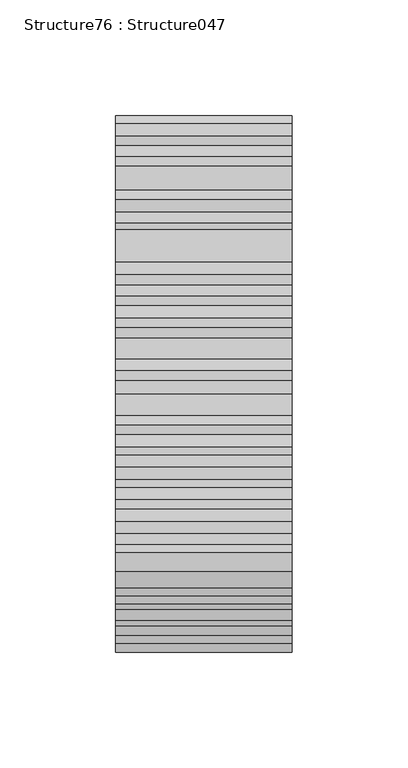
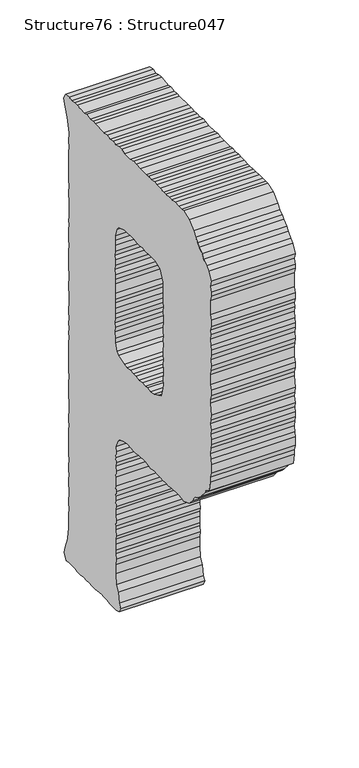
"""IFC4 building model written with IfcOpenShell, lengths in millimetres: proxy geometry, Structure76 : Structure047."""

from ifc_helpers import new_model, si_unit, frame, origin, place, context, project, spatial, polyline, outline, extrude, source, transform, mapped, element, save


def structure76_structure047_63e31db1(model_context):
    return source(origin(), model_context, "Body", "SweptSolid", [
        extrude(outline(polyline([(281300.9122556, 3996.390138), (281309.7038837, 3996.390138), (281314.3877242, 3997.5486624), (281318.4971163, 3997.5486624), (281323.7634282, 3996.390138), (281327.8647973, 3996.9645864), (281332.5566609, 3996.390138), (281337.2405014, 3996.9645864), (281342.5068134, 3996.390138), (281356.5663579, 3996.390138), (281359.5092026, 3996.9645864), (281364.1834155, 3996.390138), (281369.4673781, 3997.5486624), (281373.5687472, 3996.390138), (281384.1109987, 3997.5486624), (281388.2107632, 3997.5486624), (281392.9026268, 3996.390138), (281397.0039958, 3997.5486624), (281402.2703078, 3996.9645864), (281405.7876009, 3991.6806238), (281404.038582, 3986.4046842), (281402.2703078, 3982.8793681), (281401.0957373, 3978.2035506), (281399.3451138, 3973.5197101), (281397.0039958, 3962.9774586), (281398.1705433, 3954.7506513), (281397.0039958, 3948.917914), (281398.1705433, 3944.8165449), (281398.1705433, 3935.4328178), (281397.5864673, 3931.3346579), (281397.5864673, 3921.3748778), (281398.1705433, 3917.2735087), (281397.0039958, 3912.0071968), (281397.5864673, 3906.7328618), (281397.5864673, 3903.2059411), (281397.0039958, 3898.5301236), (281397.0039958, 3883.2863809), (281397.5864673, 3879.1769888), (281397.0039958, 3875.0772243), (281398.1705433, 3870.4030114), (281397.5864673, 3864.5446004), (281398.1705433, 3860.4432313), (281397.0039958, 3855.1769193), (281397.5864673, 3851.0595042), (281397.5864673, 3832.8921721), (281397.0039958, 3828.2163546), (281397.0039958, 3823.5341187), (281397.5864673, 3818.8310229), (281398.1705433, 3812.9726119), (281397.0039958, 3808.8888934), (281397.0039958, 3800.0876378), (281397.5864673, 3794.2292268), (281398.1705433, 3790.7039107), (281397.0039958, 3786.0280932), (281398.1705433, 3780.1616592), (281397.0039958, 3776.0618947), (281398.1705433, 3771.3860772), (281397.0039958, 3766.684586), (281397.5864673, 3762.0023501), (281397.5864673, 3756.7440611), (281398.1705433, 3752.6170184), (281398.1705433, 3743.2332913), (281397.5864673, 3739.1592005), (281398.1705433, 3733.8736333), (281397.0039958, 3729.7738688), (281397.5864673, 3723.9154578), (281397.5864673, 3720.4158154), (281398.1705433, 3715.1302482), (281397.5864673, 3709.8559132), (281397.0039958, 3705.7545441), (281397.0039958, 3696.9709391), (281397.5864673, 3691.0868544), (281397.5864673, 3686.4030139), (281397.0039958, 3682.8857208), (281397.5864673, 3678.2018803), (281398.1705433, 3672.9435914), (281397.5864673, 3668.8261762), (281397.5864673, 3662.9854159), (281398.1705433, 3658.3015753), (281398.1705433, 3654.1841602), (281397.0039958, 3650.1004418), (281398.1705433, 3644.2420307), (281397.5864673, 3639.5405396), (281397.0039958, 3635.4407751), (281397.5864673, 3630.7392839), (281397.5864673, 3626.6571701), (281397.0039958, 3620.7971545), (281397.0039958, 3616.0972679), (281398.1705433, 3612.0135494), (281398.1705433, 3607.8961343), (281397.0039958, 3602.6298224), (281398.1705433, 3597.9540049), (281398.1705433, 3593.8285667), (281397.5864673, 3588.5702778), (281397.5864673, 3584.4689087), (281399.3451138, 3573.9266571), (281399.9372129, 3570.4109687), (281402.2703078, 3564.54293), (281404.038582, 3559.8671125), (281405.1955018, 3556.3417965), (281401.6878364, 3550.4833855), (281397.5864673, 3551.0658569), (281387.6282918, 3551.0658569), (281384.1109987, 3550.4833855), (281379.4191352, 3550.4833855), (281374.1512186, 3551.0658569), (281369.4673781, 3550.4833855), (281365.3595906, 3551.0658569), (281360.6757501, 3550.4833855), (281356.5663579, 3550.4833855), (281346.0241064, 3551.6675836), (281342.5068134, 3551.6675836), (281338.4070489, 3551.0658569), (281333.1391323, 3550.4833855), (281323.1713292, 3550.4833855), (281318.4971163, 3551.6675836), (281316.1463707, 3556.3417965), (281318.4971163, 3559.8671125), (281320.2477398, 3569.2524442), (281323.1713292, 3575.0851816), (281324.3475043, 3584.4689087), (281324.3475043, 3593.2541183), (281323.1713292, 3599.1125293), (281324.3475043, 3603.7963698), (281323.7634282, 3607.3393366), (281324.3475043, 3613.1720739), (281324.3475043, 3617.8559144), (281323.1713292, 3621.3732075), (281324.3475043, 3626.6571701), (281323.7634282, 3630.7392839), (281323.1713292, 3636.0408972), (281324.3475043, 3640.7167147), (281324.3475043, 3645.9830266), (281323.1713292, 3649.5003197), (281323.7634282, 3654.7842823), (281323.7634282, 3659.4584952), (281323.1713292, 3664.1423357), (281323.7634282, 3668.8261762), (281323.7634282, 3677.6274319), (281323.1713292, 3683.4858429), (281324.3475043, 3687.587212), (281323.1713292, 3691.6869765), (281323.7634282, 3696.3884676), (281323.1713292, 3702.229228), (281324.3475043, 3706.3289925), (281320.8302112, 3713.9556777), (281318.4971163, 3716.8985223), (281310.8720357, 3719.2316172), (281305.0120201, 3720.4158154), (281300.3201566, 3719.8140887), (281296.2203921, 3719.8140887), (281292.1286506, 3719.2316172), (281286.852711, 3720.4158154), (281278.0514554, 3720.4158154), (281272.2010674, 3719.8140887), (281268.6837743, 3719.2316172), (281263.4078347, 3720.4158154), (281259.3080703, 3719.8140887), (281253.4496592, 3719.8140887), (281249.9403892, 3719.2316172), (281245.2485257, 3719.8140887), (281240.5566621, 3719.2316172), (281235.8808446, 3720.4158154), (281225.9050185, 3720.4158154), (281220.6387065, 3719.8140887), (281217.1294365, 3719.2316172), (281208.9202799, 3722.1568112), (281204.8205154, 3726.8566978), (281198.9524768, 3733.8736333), (281194.2782639, 3736.2163558), (281191.3354192, 3739.1592005), (281184.3104607, 3747.3587295), (281181.9677382, 3750.8583719), (281177.2758746, 3753.2171405), (281175.5268557, 3762.5848215), (281175.5268557, 3767.2590344), (281174.3506806, 3771.9605256), (281174.3506806, 3780.1616592), (281174.9347567, 3784.8438951), (281175.5268557, 3790.1294623), (281174.9347567, 3795.4037973), (281174.3506806, 3799.5051664), (281174.3506806, 3804.1890069), (281174.9347567, 3808.8888934), (281174.3506806, 3812.9726119), (281175.5268557, 3818.8310229), (281174.9347567, 3822.348316), (281174.3506806, 3827.6162325), (281175.5268557, 3838.1761347), (281175.5268557, 3841.6741725), (281174.3506806, 3846.3772683), (281174.3506806, 3851.6612309), (281175.5268557, 3856.3161885), (281175.5268557, 3865.7015202), (281174.9347567, 3869.8189354), (281174.3506806, 3874.5043805), (281174.9347567, 3880.3627915), (281174.3506806, 3885.0626781), (281174.3506806, 3889.7208449), (281174.9347567, 3893.822214), (281175.5268557, 3899.7046941), (281174.9347567, 3904.3901392), (281175.5268557, 3908.46423), (281174.3506806, 3912.5896682), (281174.3506806, 3918.4480792), (281175.5268557, 3923.1319197), (281175.5268557, 3936.6186205), (281174.3506806, 3941.8753048), (281174.3506806, 3945.4182716), (281175.5268557, 3950.6765605), (281174.3506806, 3955.9348494), (281177.8663691, 3963.5615346), (281181.3852667, 3966.5043792), (281185.4850312, 3970.5768654), (281187.8277538, 3974.1214368), (281192.5099897, 3977.6194746), (281194.8607353, 3980.5623192), (281198.3780283, 3983.4794902), (281201.8953214, 3987.5792547), (281208.9202799, 3994.0233463), (281217.1294365, 3997.5486624), (281220.6387065, 3996.9645864), (281225.322547, 3996.9645864), (281230.596882, 3997.5486624), (281235.8808446, 3996.9645864), (281239.9645631, 3996.9645864), (281245.2485257, 3996.390138), (281248.7577957, 3996.390138), (281254.0417583, 3996.9645864), (281259.3080703, 3996.9645864), (281262.8173403, 3997.5486624), (281268.1013029, 3996.390138), (281272.2010674, 3997.5486624), (281276.3008319, 3996.390138), (281285.6685129, 3996.390138), (281291.5365516, 3996.9645864), (281295.6443391, 3997.5486624), (281300.9122556, 3996.390138)]), holes=[polyline([(281319.0715647, 3797.1463977), (281321.4223103, 3799.5051664), (281324.3475043, 3805.9476534), (281324.3475043, 3810.6298893), (281324.9299757, 3816.4883003), (281324.3475043, 3821.1737455), (281324.9299757, 3824.7167122), (281323.7634282, 3829.9733965), (281324.3475043, 3834.0474873), (281323.7634282, 3839.3587282), (281324.3475043, 3844.6154125), (281323.7634282, 3848.1166595), (281324.3475043, 3853.4198774), (281324.3475043, 3862.8036045), (281323.7634282, 3867.4601667), (281323.7634282, 3871.5599312), (281324.9299757, 3876.263027), (281324.3475043, 3880.3627915), (281323.7634282, 3886.2051565), (281324.9299757, 3889.7208449), (281323.7634282, 3894.4030808), (281323.7634282, 3899.7046941), (281324.3475043, 3904.3901392), (281323.7634282, 3909.0627475), (281322.0047817, 3916.0909152), (281319.0715647, 3919.6066036), (281310.2879597, 3922.5494483), (281295.6443391, 3922.5494483), (281290.9524755, 3921.9733953), (281287.4351825, 3921.3748778), (281282.1608475, 3922.5494483), (281278.0514554, 3921.3748778), (281272.2010674, 3921.9733953), (281262.8173403, 3921.9733953), (281255.1986781, 3919.0321552), (281253.4496592, 3915.5068392), (281250.5244652, 3909.0627475), (281249.9403892, 3904.3901392), (281250.5244652, 3900.2887701), (281249.9403892, 3895.0048075), (281250.5244652, 3889.7208449), (281249.3498948, 3886.2051565), (281250.5244652, 3880.9452629), (281249.3498948, 3876.263027), (281249.3498948, 3870.9790644), (281249.9403892, 3866.3032469), (281249.9403892, 3862.2018778), (281249.3498948, 3857.5019912), (281250.5244652, 3854.0007442), (281249.3498948, 3848.7167816), (281250.5244652, 3844.0345457), (281249.9403892, 3839.3587282), (281249.3498948, 3835.2332901), (281249.9403892, 3830.5574726), (281249.3498948, 3825.849563), (281249.3498948, 3821.1737455), (281250.5244652, 3816.4883003), (281249.3498948, 3810.6298893), (281250.5244652, 3807.1045732), (281252.2734841, 3798.9050443), (281256.3828763, 3797.1463977), (281263.4078347, 3793.6451507), (281268.6837743, 3793.0723069), (281273.3756379, 3793.6451507), (281276.8929309, 3793.0723069), (281281.5687484, 3793.6451507), (281286.852711, 3793.0723069), (281292.1286506, 3793.6451507), (281295.6443391, 3793.6451507), (281300.3201566, 3794.2292268), (281305.5960961, 3793.6451507), (281309.7038837, 3794.2292268), (281319.0715647, 3797.1463977)])]), frame((-59031.6926606, 0.0, 0.0), z_axis=(1.0, 0.0, 0.0), x_axis=(0.0, 1.0, 0.0)), (0.0, 0.0, 1.0), 76.2),
    ])


if __name__ == "__main__":
    model = new_model("IFC4")
    model_context = context("Model", 3, world=origin())
    ifc_project = project(units=[si_unit("LENGTHUNIT", "METRE", prefix="MILLI")], contexts=[model_context])
    site = spatial("IfcSite", under=ifc_project)
    building = spatial("IfcBuilding", under=site)
    placement = place(None, origin())
    structure76_structure047_shape = structure76_structure047_63e31db1(model_context)
    element("IfcBuildingElementProxy", 1, Name="Structure76 : Structure047", ObjectType="Structure76 : Structure047", at=placement, inside=building, context=model_context, shape_type="MappedRepresentation", body=[
        mapped(structure76_structure047_shape, transform((0.0, 0.0, 0.0), x_axis=(1.0, 0.0, 0.0), y_axis=(0.0, 1.0, 0.0), z_axis=(0.0, 0.0, 1.0))),
    ])
    save(model, "model.ifc")

# Revit data of these elements
# Type "Structure76 : Structure047"
#   NameOverride = "Structure047"
# Element 1 (IfcBuildingElementProxy, "Structure76 : Structure047")
#   Materials on its faces: "BRUSHED ALUM. LETTERING"
# Materials
#   "BRUSHED ALUM. LETTERING": class "Unassigned", colour RGB 169 181 186, transparency 0, Cost = 0
